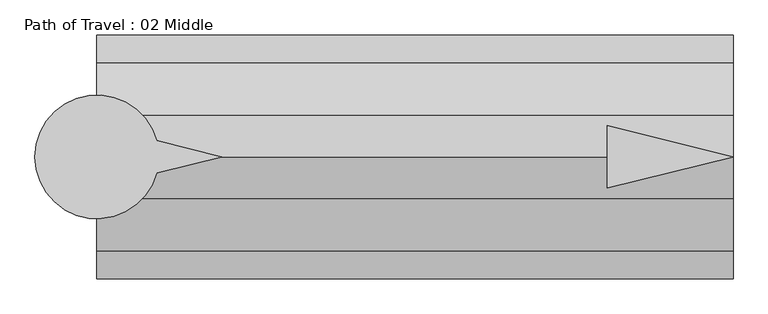
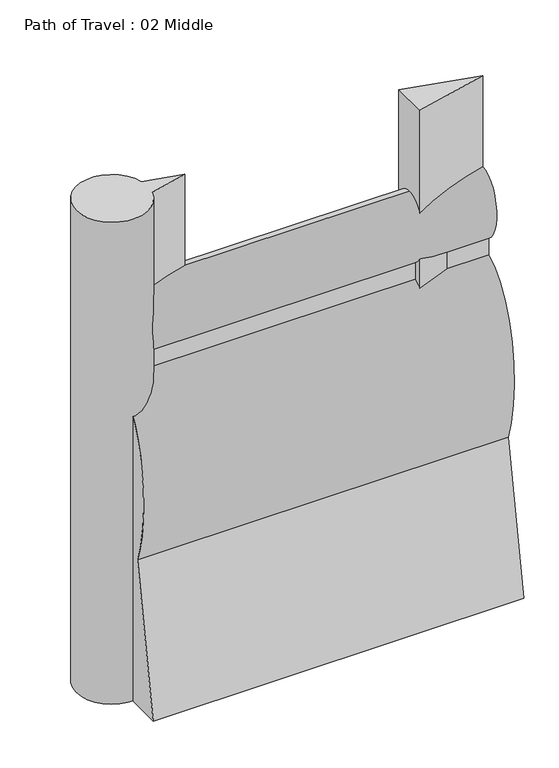
"""IFC4 building model written with IfcOpenShell, lengths in millimetres: proxy geometry, Path of Travel : 02 Middle."""

from ifc_helpers import new_model, si_unit, point, frame, frame_2d, origin, origin_with_axes, place, context, project, spatial, polyline, circle_curve, ellipse_curve, trimmed, segment, composite_curve, outline, extrude, source, transform, mapped, element, save
from ifc_brep_helpers import plane_surface, extruded_surface, advanced_brep


def path_of_travel_02_middle_d2891104(model_context):
    return source(origin(), model_context, "Body", "SolidModel", [
        advanced_brep(
        [(227.5554837, 0.0, 1727.2), (227.5554837, 42.9018657, 1436.6534209), (227.5554837, 42.9018657, 1363.4763406), (227.5554837, 184.1186263, 643.4144547), (227.5554837, 297.5699544, 0.0), (227.5554837, 145.6574193, 0.0), (227.5554837, 0.0, 584.2), (227.5554837, -145.6574193, 0.0), (227.5554837, -297.5699544, 0.0), (227.5554837, -184.1186263, 643.4144547), (227.5554837, -42.9018657, 1363.4763406), (227.5554837, -42.9018657, 1436.6534209), (1776.3129631, 0.0, 1727.2), (1776.3129631, -42.9018657, 1436.6534209), (1776.3129631, -42.9018657, 1363.4763406), (1776.3129631, -184.1186263, 643.4144547), (1776.3129631, -297.5699544, 0.0), (1776.3129631, -145.6574193, 0.0), (1776.3129631, 0.0, 584.2), (1776.3129631, 145.6574193, 0.0), (1776.3129631, 297.5699544, 0.0), (1776.3129631, 184.1186263, 643.4144547), (1776.3129631, 42.9018657, 1363.4763406), (1776.3129631, 42.9018657, 1436.6534209)],
        [
            (0, 1, ellipse_curve(frame((227.5554837, 0.0, 1574.8), z_axis=(-1.0, 0.0, 0.0), x_axis=(0.0, 0.0, 1.0)), 152.4, 101.6)),
            (1, 2),
            (2, 3, ellipse_curve(frame((227.5554837, 0.0, 914.4), z_axis=(-1.0, 0.0, 0.0), x_axis=(0.0, 0.0, -1.0)), 457.2, 228.6)),
            (3, 4),
            (4, 5),
            (5, 6),
            (6, 7),
            (7, 8),
            (8, 9),
            (9, 10, ellipse_curve(frame((227.5554837, 0.0, 914.4), z_axis=(-1.0, 0.0, 0.0), x_axis=(0.0, 0.0, -1.0)), 457.2, 228.6)),
            (10, 11),
            (11, 0, ellipse_curve(frame((227.5554837, 0.0, 1574.8), z_axis=(-1.0, 0.0, 0.0), x_axis=(0.0, 0.0, 1.0)), 152.4, 101.6)),
            (12, 13, ellipse_curve(frame((1776.3129631, 0.0, 1574.8), z_axis=(1.0, 0.0, 0.0), x_axis=(0.0, 0.0, 1.0)), 152.4, 101.6)),
            (13, 14),
            (14, 15, ellipse_curve(frame((1776.3129631, 0.0, 914.4), z_axis=(1.0, 0.0, 0.0), x_axis=(0.0, 0.0, -1.0)), 457.2, 228.6)),
            (15, 16),
            (16, 17),
            (17, 18),
            (18, 19),
            (19, 20),
            (20, 21),
            (21, 22, ellipse_curve(frame((1776.3129631, 0.0, 914.4), z_axis=(1.0, 0.0, 0.0), x_axis=(0.0, 0.0, -1.0)), 457.2, 228.6)),
            (22, 23),
            (23, 12, ellipse_curve(frame((1776.3129631, 0.0, 1574.8), z_axis=(1.0, 0.0, 0.0), x_axis=(0.0, 0.0, 1.0)), 152.4, 101.6)),
            (0, 12),
            (23, 1),
            (22, 2),
            (21, 3),
            (20, 4),
            (19, 5),
            (18, 6),
            (17, 7),
            (16, 8),
            (15, 9),
            (14, 10),
            (13, 11),
        ],
        [
            plane_surface(frame((227.5554837, 0.0, 0.0), z_axis=(-1.0, 0.0, 0.0), x_axis=(0.0, 0.0, 1.0))),
            plane_surface(frame((1776.3129631, 0.0, 0.0), z_axis=(1.0, 0.0, 0.0), x_axis=(0.0, 0.0, 1.0))),
            extruded_surface(trimmed(ellipse_curve(frame((1776.3129631, 0.0, 1574.8), z_axis=(-1.0, 0.0, 0.0), x_axis=(0.0, 0.0, 1.0)), 152.4, 101.6), [point((1776.3129631, 0.0, 1727.2))], [point((1776.3129631, 42.9018657, 1436.6534209))], True, "CARTESIAN"), (-1548.7574794, 0.0, 0.0), 1548.7574794),
            plane_surface(frame((227.5554837, 42.9018657, 1436.6534209), z_axis=(0.0, 1.0, 0.0), x_axis=(1.0, 0.0, 0.0))),
            extruded_surface(trimmed(ellipse_curve(frame((1776.3129631, 0.0, 914.4), z_axis=(-1.0, 0.0, 0.0), x_axis=(0.0, 0.0, -1.0)), 457.2, 228.6), [point((1776.3129631, 42.9018657, 1363.4763406))], [point((1776.3129631, 184.1186263, 643.4144547))], True, "CARTESIAN"), (-1548.7574794, 0.0, 0.0), 1548.7574794),
            plane_surface(frame((227.5554837, 184.1186263, 643.4144547), z_axis=(0.0, 0.9848077530122078, 0.1736481776669322), x_axis=(1.0, 0.0, 0.0))),
            plane_surface(frame((227.5554837, 297.5699544, 0.0), z_axis=(0.0, 0.0, -1.0), x_axis=(1.0, 0.0, 0.0))),
            plane_surface(frame((227.5554837, 145.6574193, 0.0), z_axis=(0.0, -0.9702957262760199, -0.2419218955995739), x_axis=(1.0, 0.0, 0.0))),
            plane_surface(frame((227.5554837, 0.0, 584.2), z_axis=(0.0, 0.9702957262759961, -0.24192189559966923), x_axis=(1.0, 0.0, 0.0))),
            plane_surface(frame((227.5554837, -145.6574193, 0.0), z_axis=(0.0, 0.0, -1.0), x_axis=(1.0, 0.0, 0.0))),
            plane_surface(frame((227.5554837, -297.5699544, 0.0), z_axis=(0.0, -0.984807753012208, 0.17364817766693066), x_axis=(1.0, 0.0, 0.0))),
            extruded_surface(trimmed(ellipse_curve(frame((1776.3129631, 0.0, 914.4), z_axis=(-1.0, 0.0, 0.0), x_axis=(0.0, 0.0, -1.0)), 457.2, 228.6), [point((1776.3129631, -184.1186263, 643.4144547))], [point((1776.3129631, -42.9018657, 1363.4763406))], True, "CARTESIAN"), (-1548.7574794, 0.0, 0.0), 1548.7574794),
            plane_surface(frame((227.5554837, -42.9018657, 1363.4763406), z_axis=(0.0, -1.0, 0.0), x_axis=(1.0, 0.0, 0.0))),
            extruded_surface(trimmed(ellipse_curve(frame((1776.3129631, 0.0, 1574.8), z_axis=(-1.0, 0.0, 0.0), x_axis=(0.0, 0.0, 1.0)), 152.4, 101.6), [point((1776.3129631, -42.9018657, 1436.6534209))], [point((1776.3129631, 0.0, 1727.2))], True, "CARTESIAN"), (-1548.7574794, 0.0, 0.0), 1548.7574794),
        ],
        [
            (0, [[1, 2, 3, 4, 5, 6, 7, 8, 9, 10, 11, 12]]),
            (1, [[13, 14, 15, 16, 17, 18, 19, 20, 21, 22, 23, 24]]),
            (2, [[-1, 25, -24, 26]]),
            (3, [[-2, -26, -23, 27]]),
            (4, [[-3, -27, -22, 28]]),
            (5, [[-4, -28, -21, 29]]),
            (6, [[-5, -29, -20, 30]]),
            (7, [[-6, -30, -19, 31]]),
            (8, [[-7, -31, -18, 32]]),
            (9, [[-8, -32, -17, 33]]),
            (10, [[-9, -33, -16, 34]]),
            (11, [[-10, -34, -15, 35]]),
            (12, [[-11, -35, -14, 36]]),
            (13, [[-12, -36, -13, -25]]),
        ],
    ),
        extrude(outline(polyline([(1470.3078166, 76.2006338), (1776.3129631, 0.0), (1470.3078166, -76.2006338), (1470.3078166, 76.2006338)])), origin_with_axes(), (0.0, 0.0, 1.0), 2129.5973753),
        extrude(outline(composite_curve([segment(polyline([(372.7837828, 39.4440225), (531.182385, 0.0), (372.7837828, -39.4440225)]), True, "CONTINUOUS"), segment(trimmed(circle_curve(frame_2d((227.2200886, 0.0)), 150.8131956), [point((372.7837828, -39.4440225))], [point((372.7837828, 39.4440225))], False, "CARTESIAN"), True, "CONTINUOUS")], self_intersect=False)), origin_with_axes(), (0.0, 0.0, 1.0), 2129.5973753),
    ])


if __name__ == "__main__":
    model = new_model("IFC4")
    model_context = context("Model", 3, world=origin())
    ifc_project = project(units=[si_unit("LENGTHUNIT", "METRE", prefix="MILLI")], contexts=[model_context])
    site = spatial("IfcSite", under=ifc_project)
    building = spatial("IfcBuilding", under=site)
    placement = place(None, origin())
    path_of_travel_02_middle_shape = path_of_travel_02_middle_d2891104(model_context)
    element("IfcBuildingElementProxy", 1, Name="Path of Travel : 02 Middle", ObjectType="Path of Travel : 02 Middle", at=placement, inside=building, context=model_context, shape_type="MappedRepresentation", body=[
        mapped(path_of_travel_02_middle_shape, transform((0.0, 0.0, 0.0), x_axis=(1.0, 0.0, 0.0), y_axis=(0.0, 1.0, 0.0), z_axis=(0.0, 0.0, 1.0))),
    ])
    save(model, "model.ifc")

# Revit data of these elements
# Type "Path of Travel : 02 Middle"
#   Path of Egress [instance default] = 4' - 0"
#   built-in parameter 1001306 [instance default] = 4 (stored number, unit not read)
#   Dot at Start = no
#   Arrow in Middle = yes
#   Arrow at End = no
#   Egress Path = none
# Element 1 (IfcBuildingElementProxy, "Path of Travel : 02 Middle")
#   Path of Egress = 5' - 0.9747"
#   built-in parameter 1001306 = 5.08123 (stored number, unit not read)
#   Materials on its faces: "Egress Path Solid", "solid"
# Materials
#   "Egress Path Solid": class "Unassigned", colour RGB 255 128 64, transparency 0.75, Comments = "Rendering appearance not upgraded "
#   "solid": class "Generic", colour RGB 120 120 120, transparency 0, Cost = 0
